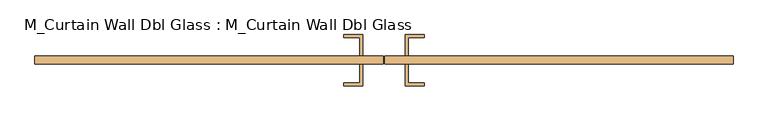
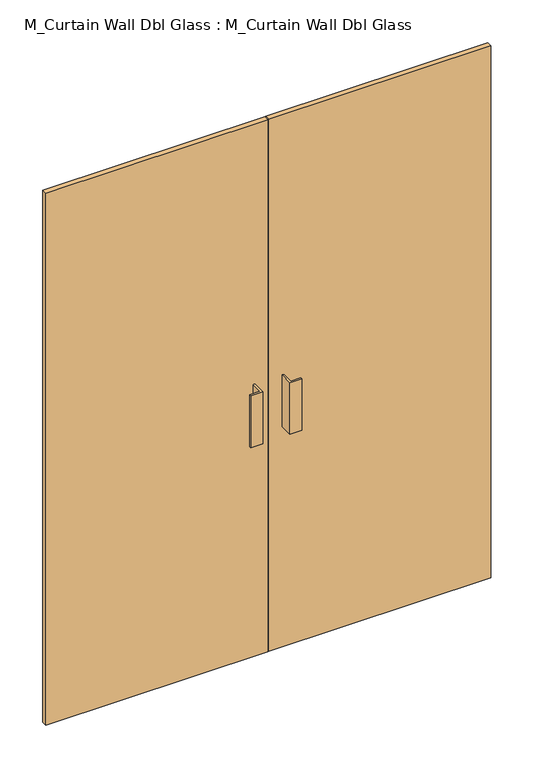
"""IFC4 building model written with IfcOpenShell, lengths in millimetres: door geometry, M_Curtain Wall Dbl Glass : M_Curtain Wall Dbl Glass."""

from ifc_helpers import new_model, si_unit, frame, origin, origin_with_axes, place, context, project, spatial, polyline, outline, extrude, source, transform, mapped, element, save


def m_curtain_wall_dbl_glass_m_curtain_wall_dbl_glass_1ae92130(model_context):
    return source(origin(), model_context, "Body", "SweptSolid", [
        extrude(outline(polyline([(-1.5875, 30.95), (-825.0, 30.95), (-825.0, 50.0), (-1.5875, 50.0), (-1.5875, 30.95)])), origin_with_axes(), (0.0, 0.0, 1.0), 2085.0),
        extrude(outline(polyline([(825.0, 30.95), (1.5875, 30.95), (1.5875, 50.0), (825.0, 50.0), (825.0, 30.95)])), origin_with_axes(), (0.0, 0.0, 1.0), 2085.0),
        extrude(outline(polyline([(-50.8, 100.8), (-50.8, 50.0), (-57.15, 50.0), (-57.15, 94.45), (-95.25, 94.45), (-95.25, 100.8), (-50.8, 100.8)])), frame((0.0, 0.0, 863.6), z_axis=(0.0, 0.0, 1.0), x_axis=(1.0, 0.0, 0.0)), (0.0, 0.0, 1.0), 203.2),
        extrude(outline(polyline([(50.8, 100.8), (95.25, 100.8), (95.25, 94.45), (57.15, 94.45), (57.15, 50.0), (50.8, 50.0), (50.8, 100.8)])), frame((0.0, 0.0, 863.6), z_axis=(0.0, 0.0, 1.0), x_axis=(1.0, 0.0, 0.0)), (0.0, 0.0, 1.0), 203.2),
        extrude(outline(polyline([(-50.8, -19.85), (-95.25, -19.85), (-95.25, -13.5), (-57.15, -13.5), (-57.15, 30.95), (-50.8, 30.95), (-50.8, -19.85)])), frame((0.0, 0.0, 863.6), z_axis=(0.0, 0.0, 1.0), x_axis=(1.0, 0.0, 0.0)), (0.0, 0.0, 1.0), 203.2),
        extrude(outline(polyline([(50.8, -19.85), (50.8, 30.95), (57.15, 30.95), (57.15, -13.5), (95.25, -13.5), (95.25, -19.85), (50.8, -19.85)])), frame((0.0, 0.0, 863.6), z_axis=(0.0, 0.0, 1.0), x_axis=(1.0, 0.0, 0.0)), (0.0, 0.0, 1.0), 203.2),
    ])


if __name__ == "__main__":
    model = new_model("IFC4")
    model_context = context("Model", 3, world=origin())
    ifc_project = project(units=[si_unit("LENGTHUNIT", "METRE", prefix="MILLI")], contexts=[model_context])
    site = spatial("IfcSite", under=ifc_project)
    building = spatial("IfcBuilding", under=site)
    placement = place(None, origin())
    m_curtain_wall_dbl_glass_m_curtain_wall_dbl_glass_shape = m_curtain_wall_dbl_glass_m_curtain_wall_dbl_glass_1ae92130(model_context)
    element("IfcDoor", 1, ObjectType="M_Curtain Wall Dbl Glass : M_Curtain Wall Dbl Glass", at=placement, inside=building, context=model_context, shape_type="MappedRepresentation", body=[
        mapped(m_curtain_wall_dbl_glass_m_curtain_wall_dbl_glass_shape, transform((0.0, 0.0, 0.0), x_axis=(1.0, 0.0, 0.0), y_axis=(0.0, 1.0, 0.0), z_axis=(0.0, 0.0, 1.0))),
    ])
    save(model, "model.ifc")

# Revit data of these elements
# Type "M_Curtain Wall Dbl Glass : M_Curtain Wall Dbl Glass"
#   Model = "12345678"
#   Manufacturer = "Dublin Doors"
#   Description = "Double Glass Door"
#   Type Mark = "41"
#   COBie.Type.CreatedBy = "design@eagle.com"
#   COBie.Type.CreatedOn = "2016-09-13T05:47:35"
#   COBie.Type.Name = "Doors_M_Curtain Wall Dbl Glass_M_Curtain Wall Dbl Glass"
#   COBie.Type.Category = "23-30 10 00 : Doors"
#   COBie.Type.Description = "Double Glass Door"
#   COBie.Type.Manufacturer = "Dublin Doors"
#   COBie.Type.ModelNumber = "12345678"
#   Construction Type Id = "GSP4R"
#   Analytic Construction = "1/8 in Pilkington single glazing"
#   COBie.Type.ReplacementCost = 0
#   Visual Light Transmittance = 0.9
#   Solar Heat Gain Coefficient = 0.78
#   Offset = 50 mm
#   Heat Transfer Coefficient (U) = 3.6886 W/(m²·K)
#   COBie.Type = yes
#   Function = 1
#   Glazing Material = Glass
# Element 1 (IfcDoor, "M_Curtain Wall Dbl Glass : M_Curtain Wall Dbl Glass")
#   Materials on its faces: "Aluminum", "Glass"
# Materials
#   "Glass": class "Glass", colour RGB 0 128 192, transparency 0.75, Description = "Soda Lime Glass", Cost = 0
#   "Aluminum": class "Metal", colour RGB 247 247 247, transparency 0, Description = "Aluminum 6061", Cost = 0
